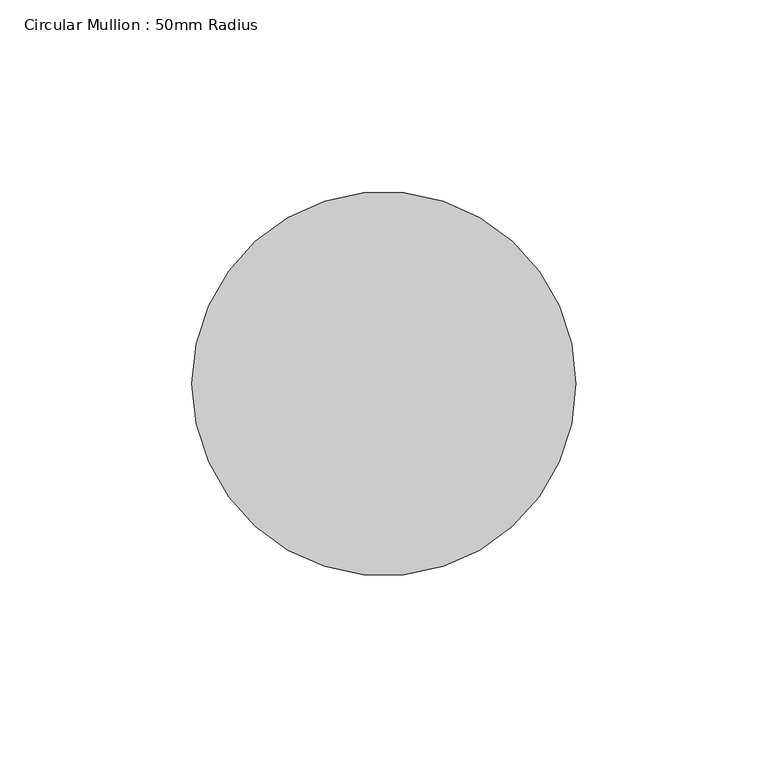
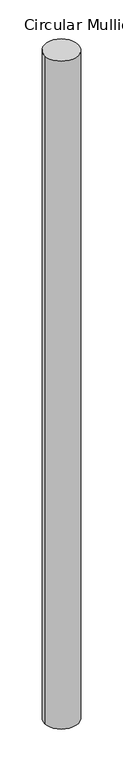
"""IFC4 building model written with IfcOpenShell, lengths in millimetres: member geometry, Circular Mullion : 50mm Radius."""

from ifc_helpers import new_model, si_unit, point, frame, frame_2d, origin, place, context, project, spatial, circle_curve, trimmed, segment, composite_curve, outline, extrude, source, transform, mapped, element, save


def circular_mullion_50mm_radius_358cfae8(model_context):
    return source(origin(), model_context, "Body", "SweptSolid", [
        extrude(outline(composite_curve([segment(trimmed(circle_curve(frame_2d((-50.0, 0.0)), 50.0), [point((0.0, 0.0))], [point((-100.0, 0.0))], False, "CARTESIAN"), True, "CONTINUOUS"), segment(trimmed(circle_curve(frame_2d((-50.0, 0.0)), 50.0), [point((-100.0, 0.0))], [point((0.0, 0.0))], False, "CARTESIAN"), True, "CONTINUOUS")], self_intersect=False)), frame((0.0, 0.0, -2105.879892), z_axis=(0.0, 0.0, 1.0), x_axis=(1.0, 0.0, 0.0)), (0.0, 0.0, 1.0), 2105.879892),
    ])


if __name__ == "__main__":
    model = new_model("IFC4")
    model_context = context("Model", 3, world=origin())
    ifc_project = project(units=[si_unit("LENGTHUNIT", "METRE", prefix="MILLI")], contexts=[model_context])
    site = spatial("IfcSite", under=ifc_project)
    building = spatial("IfcBuilding", under=site)
    placement = place(None, origin())
    circular_mullion_50mm_radius_shape = circular_mullion_50mm_radius_358cfae8(model_context)
    element("IfcMember", 1, ObjectType="Circular Mullion : 50mm Radius", at=placement, inside=building, context=model_context, shape_type="MappedRepresentation", body=[
        mapped(circular_mullion_50mm_radius_shape, transform((0.0, 0.0, 0.0), x_axis=(1.0, 0.0, 0.0), y_axis=(0.0, 1.0, 0.0), z_axis=(0.0, 0.0, 1.0))),
    ])
    save(model, "model.ifc")

# Revit data of these elements
# Type "Circular Mullion : 50mm Radius"
#   built-in parameter 1007350 = 0.164042 (stored number, unit not read)
# Element 1 (IfcMember, "Circular Mullion : 50mm Radius")
#   Materials on its faces: "Aluminium"
# Materials
#   "Aluminium": class "Metal", colour RGB 247 247 247, transparency 0, Description = "Aluminium 6061", Cost = 0
